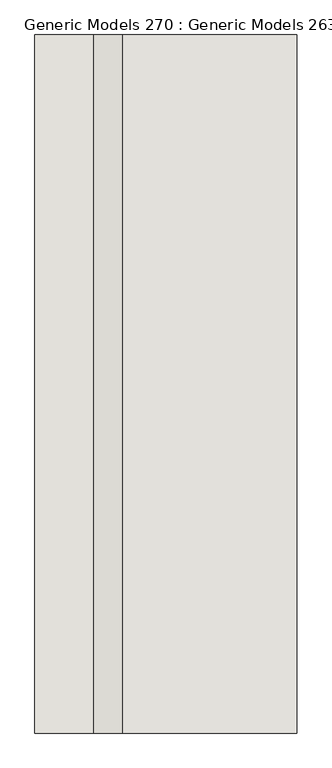
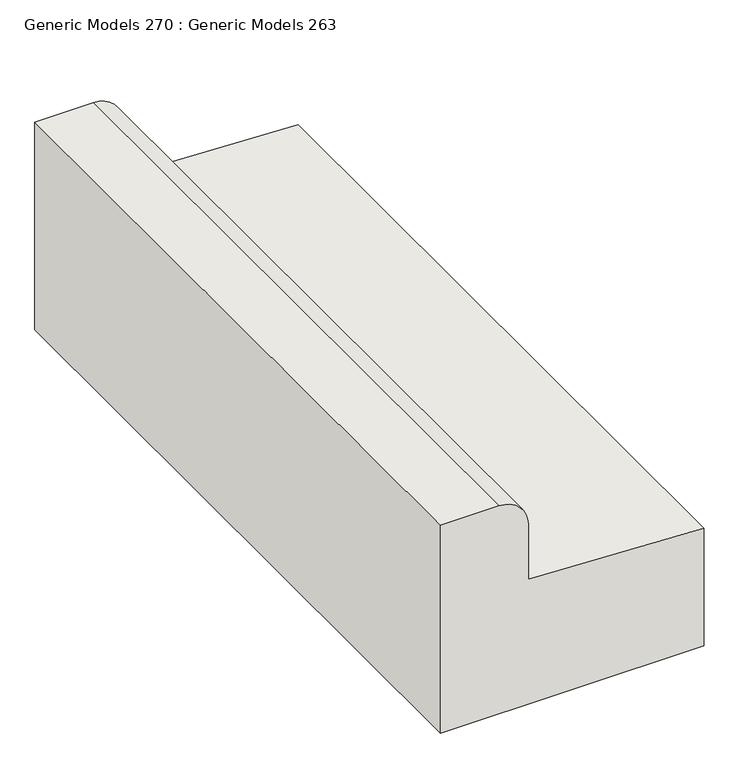
"""IFC4 building model written with IfcOpenShell, lengths in millimetres: wall geometry, Generic Models 270 : Generic Models 263."""

from ifc_helpers import new_model, si_unit, point, frame, frame_2d, origin, place, context, project, spatial, polyline, circle_curve, trimmed, segment, composite_curve, outline, extrude, source, transform, mapped, element, save


def generic_models_270_generic_models_263_c5a2dacb(model_context):
    return source(origin(), model_context, "Body", "SweptSolid", [
        extrude(outline(composite_curve([segment(polyline([(0.0, 62420.7797726), (0.0, 62319.1797726), (-381.0, 62319.1797726), (-381.0, 62776.3797726), (-165.1, 62776.3797726), (-152.4, 62471.5797726), (-50.8, 62471.5797726)]), True, "CONTINUOUS"), segment(trimmed(circle_curve(frame_2d((-50.8, 62420.7797726)), 50.8), [point((-50.8, 62471.5797726))], [point((0.0, 62420.7797726))], False, "CARTESIAN"), True, "CONTINUOUS")], self_intersect=False)), frame((0.0, -94.4486541, 0.0), z_axis=(0.0, 1.0, 0.0), x_axis=(0.0, 0.0, 1.0)), (0.0, 0.0, 1.0), 1219.2),
    ])


if __name__ == "__main__":
    model = new_model("IFC4")
    model_context = context("Model", 3, world=origin())
    ifc_project = project(units=[si_unit("LENGTHUNIT", "METRE", prefix="MILLI")], contexts=[model_context])
    site = spatial("IfcSite", under=ifc_project)
    building = spatial("IfcBuilding", under=site)
    placement = place(None, origin())
    generic_models_270_generic_models_263_shape = generic_models_270_generic_models_263_c5a2dacb(model_context)
    element("IfcWall", 1, ObjectType="Generic Models 270 : Generic Models 263", at=placement, inside=building, context=model_context, shape_type="MappedRepresentation", body=[
        mapped(generic_models_270_generic_models_263_shape, transform((0.0, 0.0, 0.0), x_axis=(1.0, 0.0, 0.0), y_axis=(0.0, 1.0, 0.0), z_axis=(0.0, 0.0, 1.0))),
    ])
    save(model, "model.ifc")

# Revit data of these elements
# Element 1 (IfcWall, "Generic Models 270 : Generic Models 263")
#   Materials on its faces: "CONCRETE CURB"
# Materials
#   "CONCRETE CURB": class "Concrete", colour RGB 191 191 191, transparency 0, Description = "Cast-in-place concrete", Cost = 0
